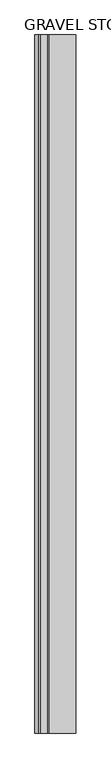
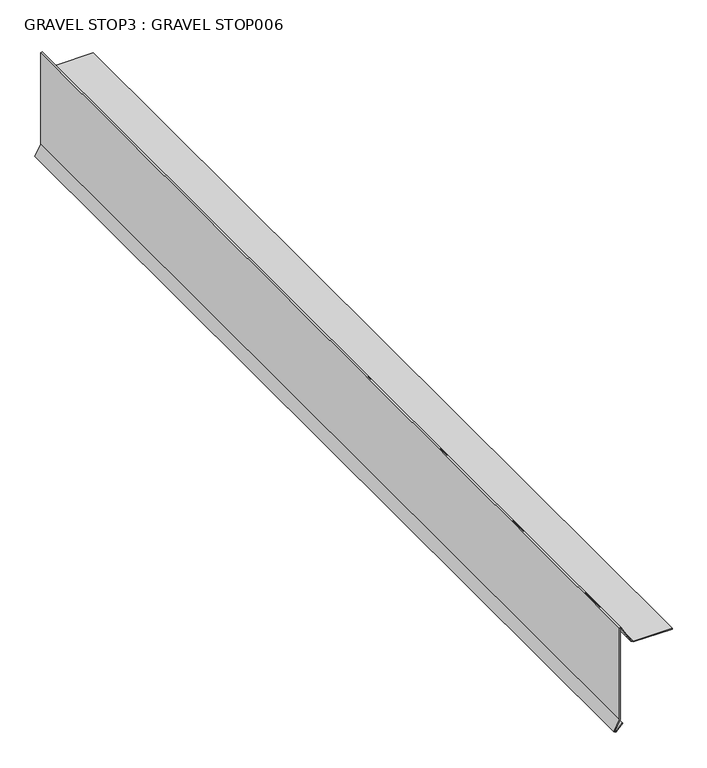
"""IFC4 building model written with IfcOpenShell, lengths in millimetres: proxy geometry, GRAVEL STOP3 : GRAVEL STOP006."""

from ifc_helpers import new_model, si_unit, frame, origin, place, context, project, spatial, polyline, outline, extrude, source, transform, mapped, element, save


def gravel_stop3_gravel_stop006_072a6e35(model_context):
    return source(origin(), model_context, "Body", "SweptSolid", [
        extrude(outline(polyline([(40077.410403, -2814.9855343), (40091.8049, -2800.5910374), (40092.8027062, -2801.5888435), (40079.2807815, -2815.1107682), (40080.9054201, -2817.2404183), (40101.495749, -2805.9993985), (40293.447969, -2805.9993985), (40293.699878, -2805.0592614), (40258.5078708, -2784.7411466), (40255.9633674, -2780.3339375), (40255.9633674, -2702.4979247), (40257.3744784, -2702.4979247), (40257.3744784, -2779.9558314), (40259.5408757, -2783.7081416), (40295.3431515, -2804.3785952), (40294.5307525, -2807.4105095), (40101.8558531, -2807.4105095), (40080.5182783, -2819.0594785), (40077.410403, -2814.9855343)])), frame((0.0, 999.75, 0.0), z_axis=(0.0, 1.0, 0.0), x_axis=(0.0, 0.0, 1.0)), (0.0, 0.0, 1.0), 2000.25),
    ])


if __name__ == "__main__":
    model = new_model("IFC4")
    model_context = context("Model", 3, world=origin())
    ifc_project = project(units=[si_unit("LENGTHUNIT", "METRE", prefix="MILLI")], contexts=[model_context])
    site = spatial("IfcSite", under=ifc_project)
    building = spatial("IfcBuilding", under=site)
    placement = place(None, origin())
    gravel_stop3_gravel_stop006_shape = gravel_stop3_gravel_stop006_072a6e35(model_context)
    element("IfcBuildingElementProxy", 1, Name="GRAVEL STOP3 : GRAVEL STOP006", ObjectType="GRAVEL STOP3 : GRAVEL STOP006", at=placement, inside=building, context=model_context, shape_type="MappedRepresentation", body=[
        mapped(gravel_stop3_gravel_stop006_shape, transform((0.0, 0.0, 0.0), x_axis=(1.0, 0.0, 0.0), y_axis=(0.0, 1.0, 0.0), z_axis=(0.0, 0.0, 1.0))),
    ])
    save(model, "model.ifc")

# Revit data of these elements
# Type "GRAVEL STOP3 : GRAVEL STOP006"
#   NameOverride = "GRAVEL STOP006"
# Element 1 (IfcBuildingElementProxy, "GRAVEL STOP3 : GRAVEL STOP006")
#   Materials on its faces: "GRAVEL STOP REQUIRED WITH GRAVEL SURFACE SYSTEMS"
# Materials
#   "GRAVEL STOP REQUIRED WITH GRAVEL SURFACE SYSTEMS": class "Unassigned", colour RGB 170 170 127, transparency 0, Cost = 0
